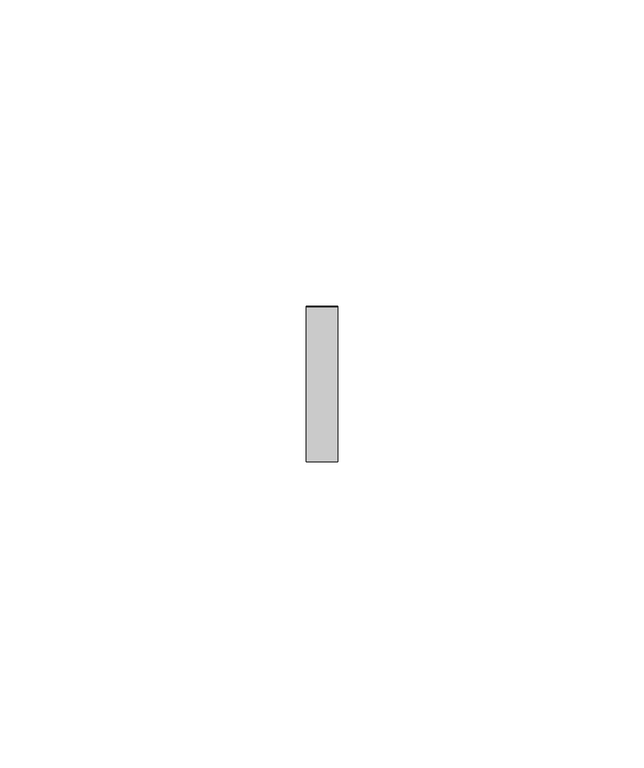
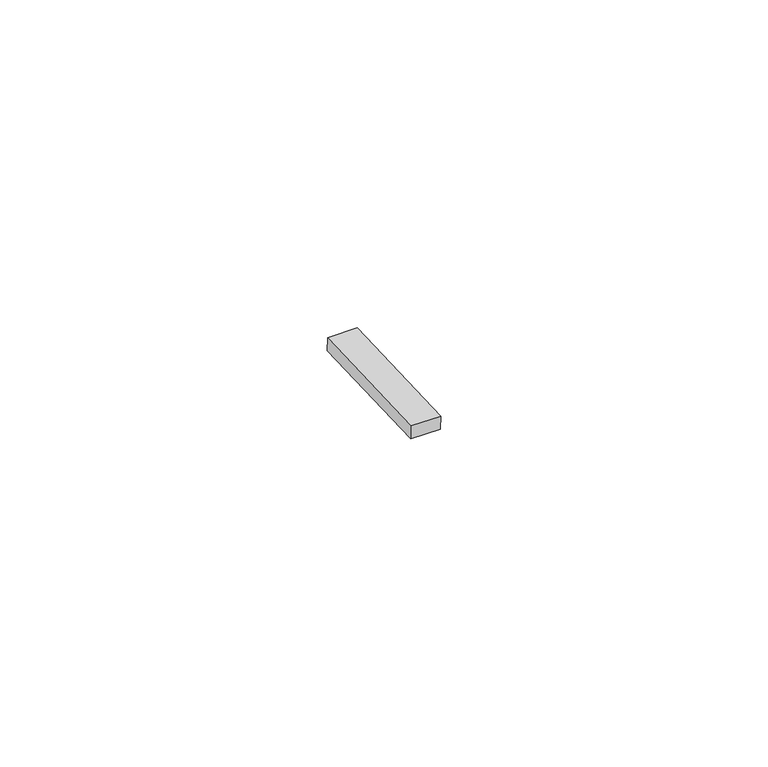
"""IFC4 building model written with IfcOpenShell, lengths in millimetres: proxy geometry, Inner panel:Inner panel:1:Inner panel:1 : Inner panel:Inner panel:300324:2:Inner panel:1:Inner panel:1 : Inner panel:Inner panel:300324:2 : Inner panel:Inner panel:1:Inner panel:1 : Inner panel:Inner panel:300324:300043:122 : Inner panel:Inner panel:1:Inner panel:1 : Inner panel:Inner panel:300324:2:Inner panel:1:Inner panel:1 : Inner panel:Inner panel:300324:2 : Inner panel:Inner panel:1:Inner panel:1 : Inner panel:Inner panel:300324:300043:308120."""

from ifc_helpers import new_model, si_unit, frame, origin, place, context, project, spatial, polyline, outline, extrude, source, transform, mapped, element, save


def generic_models_75e061b7(model_context):
    return source(origin(), model_context, "Body", "SweptSolid", [
        extrude(outline(polyline([(0.0, -25.4), (0.0, 0.0), (5.2138089, 0.0), (5.2138089, -25.4), (0.0, -25.4)])), frame((593123.795117, -578253.2828061, 3981.0403755), z_axis=(0.0, -0.041630544712223896, 0.9991330730923502), x_axis=(-1.0, 0.0, 0.0)), (0.0, 0.0, 1.0), 2.4763745),
    ])


if __name__ == "__main__":
    model = new_model("IFC4")
    model_context = context("Model", 3, world=origin())
    ifc_project = project(units=[si_unit("LENGTHUNIT", "METRE", prefix="MILLI")], contexts=[model_context])
    site = spatial("IfcSite", under=ifc_project)
    building = spatial("IfcBuilding", under=site)
    placement = place(None, origin())
    generic_models_shape = generic_models_75e061b7(model_context)
    element("IfcBuildingElementProxy", 1, Name="Inner panel:Inner panel:1:Inner panel:1 : Inner panel:Inner panel:300324:2:Inner panel:1:Inner panel:1 : Inner panel:Inner panel:300324:2 : Inner panel:Inner panel:1:Inner panel:1 : Inner panel:Inner panel:300324:300043:122 : Inner panel:Inner panel:1:Inner panel:1 : Inner panel:Inner panel:300324:2:Inner panel:1:Inner panel:1 : Inner panel:Inner panel:300324:2 : Inner panel:Inner panel:1:Inner panel:1 : Inner panel:Inner panel:300324:300043:308120", ObjectType="Inner panel:Inner panel:1:Inner panel:1 : Inner panel:Inner panel:300324:2:Inner panel:1:Inner panel:1 : Inner panel:Inner panel:300324:2 : Inner panel:Inner panel:1:Inner panel:1 : Inner panel:Inner panel:300324:300043:122 : Inner panel:Inner panel:1:Inner panel:1 : Inner panel:Inner panel:300324:2:Inner panel:1:Inner panel:1 : Inner panel:Inner panel:300324:2 : Inner panel:Inner panel:1:Inner panel:1 : Inner panel:Inner panel:300324:300043:308120", at=placement, inside=building, context=model_context, shape_type="MappedRepresentation", body=[
        mapped(generic_models_shape, transform((0.0, 0.0, 0.0), x_axis=(1.0, 0.0, 0.0), y_axis=(0.0, 1.0, 0.0), z_axis=(0.0, 0.0, 1.0))),
    ])
    save(model, "model.ifc")

# Revit data of these elements
# Type "Inner panel:Inner panel:1:Inner panel:1 : Inner panel:Inner panel:300324:2:Inner panel:1:Inner panel:1 : Inner panel:Inner panel:300324:2 : Inner panel:Inner panel:1:Inner panel:1 : Inner panel:Inner panel:300324:300043:122 : Inner panel:Inner panel:1:Inner panel:1 : Inner panel:Inner panel:300324:2:Inner panel:1:Inner panel:1 : Inner panel:Inner panel:300324:2 : Inner panel:Inner panel:1:Inner panel:1 : Inner panel:Inner panel:300324:300043:308120"
#   NameOverride = "Inner panel:Inner panel:1:Inner panel:1 : Inner panel:Inner panel:300324:2:Inner panel:1:Inner panel:1 : Inner panel:Inner panel:300324:2 : Inner panel:Inner panel:1:Inner panel:1 : Inner panel:Inner panel:300324:300043:308120"
#   ObjectTypeOverride = "Inner panel:1:Inner panel:1 : Inner panel:Inner panel:300324:2 : Inner panel:Inner panel:1:Inner panel:1 : Inner panel:Inner panel:300324:300043"
#   Reference = "Inner panel"
#   Tag = "308120"
# Element 1 (IfcBuildingElementProxy, "Inner panel:Inner panel:1:Inner panel:1 : Inner panel:Inner panel:300324:2:Inner panel:1:Inner panel:1 : Inner panel:Inner panel:300324:2 : Inner panel:Inner panel:1:Inner panel:1 : Inner panel:Inner panel:300324:300043:122 : Inner panel:Inner panel:1:Inner panel:1 : Inner panel:Inner panel:300324:2:Inner panel:1:Inner panel:1 : Inner panel:Inner panel:300324:2 : Inner panel:Inner panel:1:Inner panel:1 : Inner panel:Inner panel:300324:300043:308120")
#   Materials on its faces: "AT CLIP - 1\" WIDE NON ABSORBENT, WEATHER-RESISTANT NEOPRENE/EPDM/SBR FOAM"
# Materials
#   "AT CLIP - 1\" WIDE NON ABSORBENT, WEATHER-RESISTANT NEOPRENE/EPDM/SBR FOAM": class "Generic", colour RGB 85 85 85, transparency 0, Cost = 0
